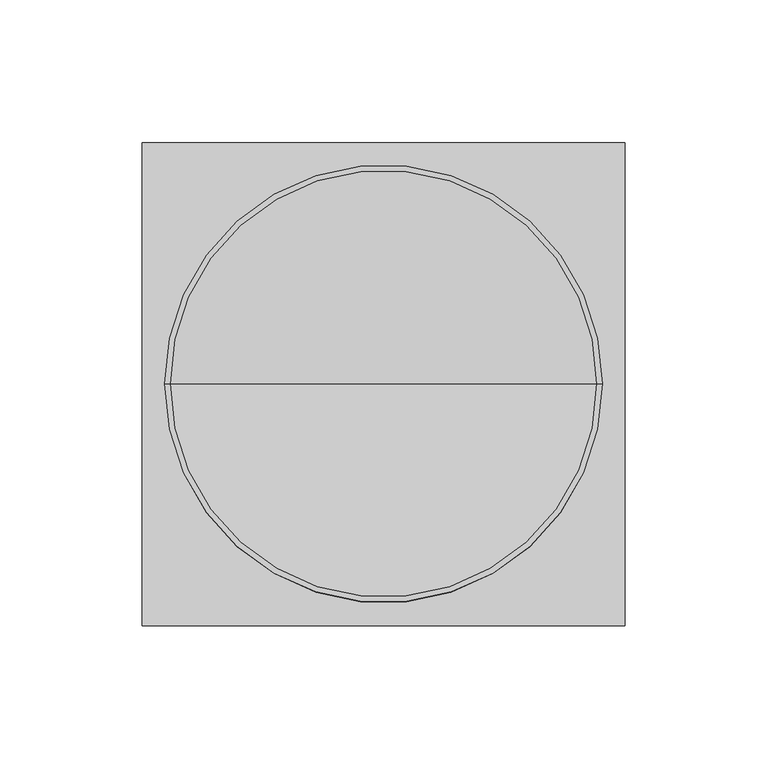
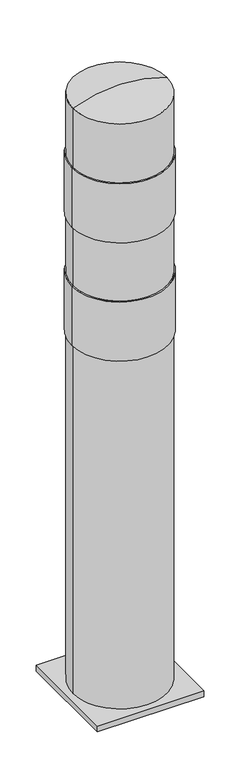
"""IFC4 building model written with IfcOpenShell, lengths in millimetres: proxy geometry, Signage_All_Loading-Systems_Safety-Bollardsrfa : H_GM_AR_B07_Steel Bollard_D150."""

from ifc_helpers import new_model, si_unit, point, frame, origin, origin_with_axes, place, context, project, spatial, polyline, circle_curve, ellipse_curve, trimmed, outline, extrude, source, transform, mapped, element, save
from ifc_brep_helpers import plane_surface, cylinder_surface, revolved_surface, advanced_brep


def generic_models_1bc9e902(model_context):
    return source(origin(), model_context, "Body", "SolidModel", [
        advanced_brep(
        [(-70.0942839, 0.0, 800.0), (-147.0942839, 0.0, 800.0), (6.9057161, 0.0, 800.0), (6.9057161, 0.0, 900.0), (-147.0942839, 0.0, 900.0), (-70.0942839, 0.0, 900.0)],
        [
            (0, 1),
            (1, 2, circle_curve(frame((-70.0942839, 0.0, 800.0), z_axis=(0.0, 0.0, -1.0), x_axis=(-1.0, 0.0, 0.0)), 77.0)),
            (2, 0),
            (2, 1, circle_curve(frame((-70.0942839, 0.0, 800.0), z_axis=(0.0, 0.0, -1.0), x_axis=(-1.0, 0.0, 0.0)), 77.0)),
            (3, 4, circle_curve(frame((-70.0942839, 0.0, 900.0), z_axis=(0.0, 0.0, 1.0), x_axis=(-1.0, 0.0, 0.0)), 77.0)),
            (4, 5),
            (5, 3),
            (4, 3, circle_curve(frame((-70.0942839, 0.0, 900.0), z_axis=(0.0, 0.0, 1.0), x_axis=(-1.0, 0.0, 0.0)), 77.0)),
            (1, 4),
            (3, 2),
        ],
        [
            plane_surface(frame((-70.0942839, 0.0, 800.0), z_axis=(0.0, 0.0, -1.0), x_axis=(-1.0, 0.0, 0.0))),
            plane_surface(frame((-70.0942839, 0.0, 900.0), z_axis=(0.0, 0.0, 1.0), x_axis=(-1.0, 0.0, 0.0))),
            cylinder_surface(frame((-70.0942839, 0.0, 1210.0), z_axis=(0.0, 0.0, -1.0), x_axis=(-1.0, 0.0, 0.0)), 77.0),
        ],
        [
            (0, [[1, 2, 3]]),
            (0, [[-3, 4, -1]]),
            (1, [[5, 6, 7]]),
            (1, [[8, -7, -6]]),
            (2, [[-2, 9, -5, 10]]),
            (2, [[-4, -10, -8, -9]]),
        ],
    ),
        advanced_brep(
        [(-70.0942839, 0.0, 600.0), (-147.0942839, 0.0, 600.0), (6.9057161, 0.0, 600.0), (6.9057161, 0.0, 700.0), (-147.0942839, 0.0, 700.0), (-70.0942839, 0.0, 700.0)],
        [
            (0, 1),
            (1, 2, circle_curve(frame((-70.0942839, 0.0, 600.0), z_axis=(0.0, 0.0, -1.0), x_axis=(-1.0, 0.0, 0.0)), 77.0)),
            (2, 0),
            (2, 1, circle_curve(frame((-70.0942839, 0.0, 600.0), z_axis=(0.0, 0.0, -1.0), x_axis=(-1.0, 0.0, 0.0)), 77.0)),
            (3, 4, circle_curve(frame((-70.0942839, 0.0, 700.0), z_axis=(0.0, 0.0, 1.0), x_axis=(-1.0, 0.0, 0.0)), 77.0)),
            (4, 5),
            (5, 3),
            (4, 3, circle_curve(frame((-70.0942839, 0.0, 700.0), z_axis=(0.0, 0.0, 1.0), x_axis=(-1.0, 0.0, 0.0)), 77.0)),
            (1, 4),
            (3, 2),
        ],
        [
            plane_surface(frame((-70.0942839, 0.0, 600.0), z_axis=(0.0, 0.0, -1.0), x_axis=(-1.0, 0.0, 0.0))),
            plane_surface(frame((-70.0942839, 0.0, 700.0), z_axis=(0.0, 0.0, 1.0), x_axis=(-1.0, 0.0, 0.0))),
            cylinder_surface(frame((-70.0942839, 0.0, 1210.0), z_axis=(0.0, 0.0, -1.0), x_axis=(-1.0, 0.0, 0.0)), 77.0),
        ],
        [
            (0, [[1, 2, 3]]),
            (0, [[-3, 4, -1]]),
            (1, [[5, 6, 7]]),
            (1, [[8, -7, -6]]),
            (2, [[-2, 9, -5, 10]]),
            (2, [[-4, -10, -8, -9]]),
        ],
    ),
        advanced_brep(
        [(4.9057161, 0.0, 600.0), (-145.0942839, 0.0, 600.0), (-70.0942839, 0.0, 600.0), (-70.0942839, 0.0, 10.0), (-145.0942839, 0.0, 10.0), (4.9057161, 0.0, 10.0)],
        [
            (0, 1, circle_curve(frame((-70.0942839, 0.0, 600.0), z_axis=(0.0, 0.0, 1.0), x_axis=(-1.0, 0.0, 0.0)), 75.0)),
            (1, 2),
            (2, 0),
            (1, 0, circle_curve(frame((-70.0942839, 0.0, 600.0), z_axis=(0.0, 0.0, 1.0), x_axis=(-1.0, 0.0, 0.0)), 75.0)),
            (3, 4),
            (4, 5, circle_curve(frame((-70.0942839, 0.0, 10.0), z_axis=(0.0, 0.0, -1.0), x_axis=(-1.0, 0.0, 0.0)), 75.0)),
            (5, 3),
            (5, 4, circle_curve(frame((-70.0942839, 0.0, 10.0), z_axis=(0.0, 0.0, -1.0), x_axis=(-1.0, 0.0, 0.0)), 75.0)),
            (4, 1),
            (0, 5),
        ],
        [
            plane_surface(frame((-70.0942839, 0.0, 600.0), z_axis=(0.0, 0.0, 1.0), x_axis=(-1.0, 0.0, 0.0))),
            plane_surface(frame((-70.0942839, 0.0, 10.0), z_axis=(0.0, 0.0, -1.0), x_axis=(-1.0, 0.0, 0.0))),
            cylinder_surface(frame((-70.0942839, 0.0, 1060.0), z_axis=(0.0, 0.0, -1.0), x_axis=(-1.0, 0.0, 0.0)), 75.0),
        ],
        [
            (0, [[1, 2, 3]]),
            (0, [[4, -3, -2]]),
            (1, [[5, 6, 7]]),
            (1, [[-7, 8, -5]]),
            (2, [[-6, 9, -1, 10]]),
            (2, [[-8, -10, -4, -9]]),
        ],
    ),
        advanced_brep(
        [(-70.0942839, 0.0, 700.0), (-145.0942839, 0.0, 700.0), (4.9057161, 0.0, 700.0), (-145.0942839, 0.0, 800.0), (4.9057161, 0.0, 800.0), (-70.0942839, 0.0, 800.0)],
        [
            (0, 1),
            (1, 2, circle_curve(frame((-70.0942839, 0.0, 700.0), z_axis=(0.0, 0.0, -1.0), x_axis=(-1.0, 0.0, 0.0)), 75.0)),
            (2, 0),
            (2, 1, circle_curve(frame((-70.0942839, 0.0, 700.0), z_axis=(0.0, 0.0, -1.0), x_axis=(-1.0, 0.0, 0.0)), 75.0)),
            (1, 3),
            (3, 4, circle_curve(frame((-70.0942839, 0.0, 800.0), z_axis=(0.0, 0.0, -1.0), x_axis=(-1.0, 0.0, 0.0)), 75.0)),
            (4, 2),
            (4, 3, circle_curve(frame((-70.0942839, 0.0, 800.0), z_axis=(0.0, 0.0, -1.0), x_axis=(-1.0, 0.0, 0.0)), 75.0)),
            (3, 5),
            (5, 4),
        ],
        [
            plane_surface(frame((-70.0942839, 0.0, 700.0), z_axis=(0.0, 0.0, -1.0), x_axis=(-1.0, 0.0, 0.0))),
            cylinder_surface(frame((-70.0942839, 0.0, 1060.0), z_axis=(0.0, 0.0, -1.0), x_axis=(-1.0, 0.0, 0.0)), 75.0),
            plane_surface(frame((-70.0942839, 0.0, 800.0), z_axis=(0.0, 0.0, 1.0), x_axis=(-1.0, 0.0, 0.0))),
        ],
        [
            (0, [[1, 2, 3]]),
            (0, [[-3, 4, -1]]),
            (1, [[-2, 5, 6, 7]]),
            (1, [[-4, -7, 8, -5]]),
            (2, [[-6, 9, 10]]),
            (2, [[-8, -10, -9]]),
        ],
    ),
        advanced_brep(
        [(4.9057161, 0.0, 1000.0), (-145.0942839, 0.0, 1000.0), (-70.0942839, 0.0, 1015.0), (-70.0942839, 0.0, 900.0), (-145.0942839, 0.0, 900.0), (4.9057161, 0.0, 900.0)],
        [
            (0, 1, circle_curve(frame((-70.0942839, 0.0, 1000.0), z_axis=(0.0, 0.0, 1.0), x_axis=(-1.0, 0.0, 0.0)), 75.0)),
            (1, 2, circle_curve(frame((-68.2073512, 0.0, 810.5653364), z_axis=(0.0, 1.0, 0.0), x_axis=(1.0, 0.0, 0.0)), 204.4433716)),
            (2, 0, circle_curve(frame((-71.9812166, 0.0, 810.5653364), z_axis=(0.0, 1.0, 0.0), x_axis=(-1.0, 0.0, 0.0)), 204.4433716)),
            (1, 0, circle_curve(frame((-70.0942839, 0.0, 1000.0), z_axis=(0.0, 0.0, 1.0), x_axis=(-1.0, 0.0, 0.0)), 75.0)),
            (3, 4),
            (4, 5, circle_curve(frame((-70.0942839, 0.0, 900.0), z_axis=(0.0, 0.0, -1.0), x_axis=(-1.0, 0.0, 0.0)), 75.0)),
            (5, 3),
            (5, 4, circle_curve(frame((-70.0942839, 0.0, 900.0), z_axis=(0.0, 0.0, -1.0), x_axis=(-1.0, 0.0, 0.0)), 75.0)),
            (4, 1),
            (0, 5),
        ],
        [
            revolved_surface(trimmed(ellipse_curve(frame((-68.2073512, 0.0, 810.5653364), z_axis=(0.0, -1.0, 0.0), x_axis=(1.0, 0.0, 0.0)), 204.4433716, 204.4433716), [point((-70.0942839, 0.0, 1015.0))], [point((-145.0942839, 0.0, 1000.0))], True, "CARTESIAN"), (-70.0942839, 0.0, 1060.0), (0.0, 0.0, -1.0)),
            plane_surface(frame((-70.0942839, 0.0, 900.0), z_axis=(0.0, 0.0, -1.0), x_axis=(-1.0, 0.0, 0.0))),
            cylinder_surface(frame((-70.0942839, 0.0, 1060.0), z_axis=(0.0, 0.0, -1.0), x_axis=(-1.0, 0.0, 0.0)), 75.0),
        ],
        [
            (0, [[1, 2, 3]]),
            (0, [[4, -3, -2]]),
            (1, [[5, 6, 7]]),
            (1, [[-7, 8, -5]]),
            (2, [[-6, 9, -1, 10]]),
            (2, [[-8, -10, -4, -9]]),
        ],
    ),
        extrude(outline(polyline([(14.9057161, 85.0), (14.9057161, -85.0), (-155.0942839, -85.0), (-155.0942839, 85.0), (14.9057161, 85.0)])), origin_with_axes(), (0.0, 0.0, 1.0), 10.0),
    ])


if __name__ == "__main__":
    model = new_model("IFC4")
    model_context = context("Model", 3, world=origin())
    ifc_project = project(units=[si_unit("LENGTHUNIT", "METRE", prefix="MILLI")], contexts=[model_context])
    site = spatial("IfcSite", under=ifc_project)
    building = spatial("IfcBuilding", under=site)
    placement = place(None, origin())
    generic_models_shape = generic_models_1bc9e902(model_context)
    element("IfcBuildingElementProxy", 1, Name="Signage_All_Loading-Systems_Safety-Bollardsrfa : H_GM_AR_B07_Steel Bollard_D150", ObjectType="Signage_All_Loading-Systems_Safety-Bollardsrfa : H_GM_AR_B07_Steel Bollard_D150", at=placement, inside=building, context=model_context, shape_type="MappedRepresentation", body=[
        mapped(generic_models_shape, transform((0.0, 0.0, 0.0), x_axis=(1.0, 0.0, 0.0), y_axis=(0.0, 1.0, 0.0), z_axis=(0.0, 0.0, 1.0))),
    ])
    save(model, "model.ifc")

# Revit data of these elements
# Type "Signage_All_Loading-Systems_Safety-Bollardsrfa : H_GM_AR_B07_Steel Bollard_D150"
#   UniFormat II Description = "Vehicular Equipment"
#   UniFormat II = "E1030"
#   UniClass 2.0 Description = "Stainless Steel Bollards"
#   UniClass 2.0 = "Pr_20_76_08_82"
#   UniClass 1.4 Description = "Bollards"
#   UniClass 1.4 = "L8111"
#   UNSPSC Description = "Fixed traffic bollard"
#   UNSPSC = "46161533"
#   NBS Reference Description = "Stainless steel bollards"
#   NBS Reference = "45-25-15/313"
#   MasterFormat 2014 Description = "Manufactured Metal Bollards"
#   MasterFormat 2014 = "32 39 13"
#   Keynote = "32 39 13"
#   IFC Category = "Ramp"
#   Copyright = "©2018 BIM Project s.r.o."
#   COBIe Category = ""
#   URL = "http://www.loading-systems.com/"
#   Type Comments = "The new robust Loading Systems safety bollards provide optimal protection around your loading and unloading area."
#   BIM Project Category = "Loading Equipment"
#   Model = "960-051"
#   Manufacturer = "LOADING SYSTEMS"
#   Description = "Safety bollards"
#   Assembly Code = "E1030300"
#   Weight = 10.00 kg
#   Top = 15 mm
#   Length = 170 mm
#   Height = 1000 mm
#   Diameter = 150 mm
#   Depth = 170 mm
#   Default Elevation = 0
# Element 1 (IfcBuildingElementProxy, "Signage_All_Loading-Systems_Safety-Bollardsrfa : H_GM_AR_B07_Steel Bollard_D150")
#   Materials on its faces: "Paint - Yellow", "Plastic - Loading Systems - Rubber - Black"
# Materials
#   "Paint - Yellow": class "Paint", colour RGB 255 255 0, transparency 0
#   "Plastic - Loading Systems - Rubber - Black": class "Plast", colour RGB 63 63 63, transparency 0, Cost = 0
